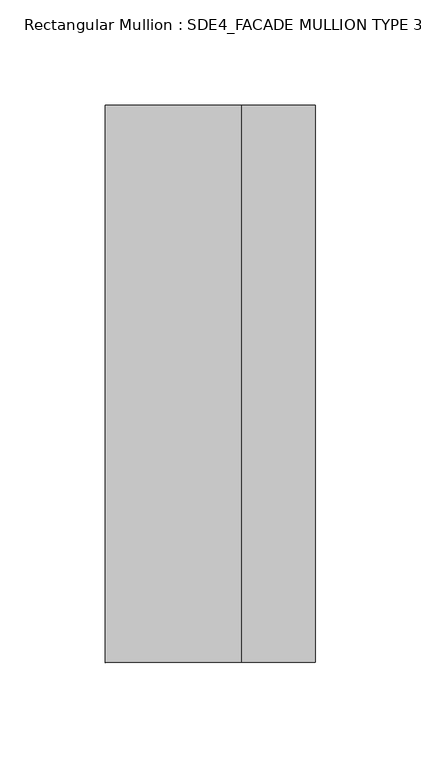
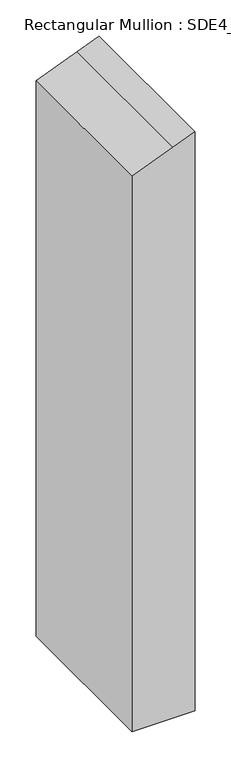
"""IFC4 building model written with IfcOpenShell, lengths in millimetres: member geometry, Rectangular Mullion : SDE4_FACADE MULLION TYPE 3."""

from ifc_helpers import new_model, si_unit, frame, origin, place, context, project, spatial, polyline, outline, extrude, source, transform, mapped, element, save


def rectangular_mullion_sde4_facade_mullion_type_3_3a96cdce(model_context):
    return source(origin(), model_context, "Body", "SweptSolid", [
        extrude(outline(polyline([(-23.0813185, 50.0), (-37.1390676, 14.8556271), (-63.0813185, -50.0), (-997.974544, -50.0), (-997.974544, 50.0), (-23.0813185, 50.0)])), frame((0.0, -132.5, 0.0), z_axis=(0.0, 1.0, 0.0), x_axis=(0.0, 0.0, 1.0)), (0.0, 0.0, 1.0), 265.0),
    ])


if __name__ == "__main__":
    model = new_model("IFC4")
    model_context = context("Model", 3, world=origin())
    ifc_project = project(units=[si_unit("LENGTHUNIT", "METRE", prefix="MILLI")], contexts=[model_context])
    site = spatial("IfcSite", under=ifc_project)
    building = spatial("IfcBuilding", under=site)
    placement = place(None, origin())
    rectangular_mullion_sde4_facade_mullion_type_3_shape = rectangular_mullion_sde4_facade_mullion_type_3_3a96cdce(model_context)
    element("IfcMember", 1, ObjectType="Rectangular Mullion : SDE4_FACADE MULLION TYPE 3", at=placement, inside=building, context=model_context, shape_type="MappedRepresentation", body=[
        mapped(rectangular_mullion_sde4_facade_mullion_type_3_shape, transform((0.0, 0.0, 0.0), x_axis=(1.0, 0.0, 0.0), y_axis=(0.0, 1.0, 0.0), z_axis=(0.0, 0.0, 1.0))),
    ])
    save(model, "model.ifc")

# Revit data of these elements
# Type "Rectangular Mullion : SDE4_FACADE MULLION TYPE 3"
#   built-in parameter 1007322 = 0.869423 (stored number, unit not read)
#   built-in parameter 1007321 = 0.164042 (stored number, unit not read)
#   built-in parameter 1007320 = 0.164042 (stored number, unit not read)
